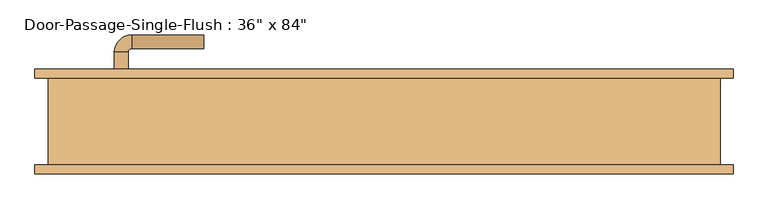
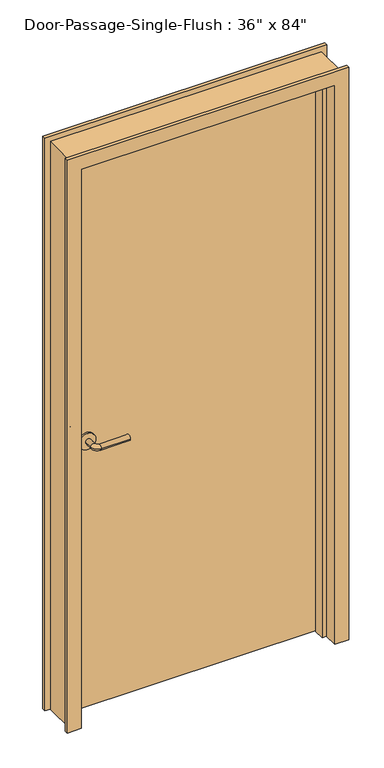
"""IFC4 building model written with IfcOpenShell, lengths in millimetres: door geometry."""

import ifcopenshell
import ifcopenshell.guid

model = None  # the IFC model being written
_history = None  # IfcOwnerHistory: only IFC2X3 demands one
_inside = {}  # id of a spatial element -> (the spatial element, [elements in it])
_under = {}  # id of a project, library or spatial element -> (it, [spatial elements below it])
_declared = {}  # id of a project -> (the project, [libraries it declares])
_typed = {}  # id of a type object -> (the type object, [elements of that type])
_made_of = {}  # id of a material, layer set ... -> (it, [elements and type objects made of it])


def new_model(schema):
    """Start an empty IFC model of exactly this schema.

    Asked for "IFC4X3", IfcOpenShell would pick the latest addendum, in which some entities
    have other attributes; the version numbers below select the first issue.
    IFC2X3 requires an IfcOwnerHistory on every rooted entity: one is made here for all.
    """
    global model, _history
    if schema == "IFC4X3":
        model = ifcopenshell.file(schema_version=(4, 3, 0, 0))
    else:
        model = ifcopenshell.file(schema=schema)
    _inside.clear()
    _under.clear()
    _declared.clear()
    _typed.clear()
    _made_of.clear()
    _history = None
    if model.schema == "IFC2X3":
        org = make("IfcOrganization", Name="unknown")
        user = make(
            "IfcPersonAndOrganization",
            ThePerson=make("IfcPerson", FamilyName="unknown"),
            TheOrganization=org,
        )
        app = make(
            "IfcApplication",
            ApplicationDeveloper=org,
            Version="unknown",
            ApplicationFullName="unknown",
            ApplicationIdentifier="unknown",
        )
        _history = make(
            "IfcOwnerHistory",
            OwningUser=user,
            OwningApplication=app,
            ChangeAction="ADDED",
            CreationDate=0,
        )
    return model


def make(cls, **values):
    """One entity of the class cls with the attributes given. An attribute that is None is left unset."""
    return model.create_entity(
        cls, **{name: value for name, value in values.items() if value is not None}
    )


def rooted(cls, **values):
    """An entity with a GlobalId (a new one), such as an element, a storey or a relation."""
    return make(cls, GlobalId=ifcopenshell.guid.new(), OwnerHistory=_history, **values)


def si_unit(unit_type, name, prefix=None):
    """IfcSIUnit, for example si_unit("LENGTHUNIT", "METRE", prefix="MILLI")."""
    return make("IfcSIUnit", UnitType=unit_type, Prefix=prefix, Name=name)


def assignment(units):
    """IfcUnitAssignment: the units of a project."""
    return None if units is None else make("IfcUnitAssignment", Units=units)


def point(xyz):
    """IfcCartesianPoint."""
    return None if xyz is None else make("IfcCartesianPoint", Coordinates=xyz)


def direction(xyz):
    """IfcDirection."""
    return None if xyz is None else make("IfcDirection", DirectionRatios=xyz)


def frame(location, z_axis=None, x_axis=None):
    """IfcAxis2Placement3D, a coordinate frame: its origin and axes. An axis left out is left unset."""
    return make(
        "IfcAxis2Placement3D",
        Location=point(location),
        Axis=direction(z_axis),
        RefDirection=direction(x_axis),
    )


def frame_2d(location, x_axis=None):
    """IfcAxis2Placement2D, a coordinate frame in the plane: its origin and x axis."""
    return make(
        "IfcAxis2Placement2D", Location=point(location), RefDirection=direction(x_axis)
    )


def origin():
    """The frame at (0, 0, 0) with its axes left unset."""
    return frame((0.0, 0.0, 0.0))


def origin_with_axes():
    """The frame at (0, 0, 0) with the z axis (0, 0, 1) and the x axis (1, 0, 0) written out."""
    return frame((0.0, 0.0, 0.0), z_axis=(0.0, 0.0, 1.0), x_axis=(1.0, 0.0, 0.0))


def place(relative_to, where):
    """IfcLocalPlacement: puts the frame where relative to a parent placement (None: the world)."""
    return make(
        "IfcLocalPlacement", PlacementRelTo=relative_to, RelativePlacement=where
    )


def context(
    kind, dimensions, precision=None, world=None, true_north=None, identifier=None
):
    """IfcGeometricRepresentationContext, for example the 3D "Model" context."""
    return make(
        "IfcGeometricRepresentationContext",
        ContextIdentifier=identifier,
        ContextType=kind,
        CoordinateSpaceDimension=dimensions,
        Precision=precision,
        WorldCoordinateSystem=world,
        TrueNorth=true_north,
    )


def project(units=None, contexts=None):
    """IfcProject with its units and contexts."""
    return rooted(
        "IfcProject",
        Name="project",
        RepresentationContexts=contexts,
        UnitsInContext=assignment(units),
    )


def spatial(cls, under=None, at=None, **own):
    """A site, building, storey or space (cls), placed at a placement, below another one or the project."""
    s = rooted(cls, ObjectPlacement=at, **own)
    if under is not None:
        _under.setdefault(under.id(), (under, []))[1].append(s)
    return s


def polyline(points):
    """IfcPolyline through the points."""
    return make("IfcPolyline", Points=[point(p) for p in points])


def circle_curve(where, radius):
    """IfcCircle in the frame where."""
    return make("IfcCircle", Position=where, Radius=radius)


def ellipse_curve(where, semi_axis1, semi_axis2):
    """IfcEllipse in the frame where."""
    return make(
        "IfcEllipse", Position=where, SemiAxis1=semi_axis1, SemiAxis2=semi_axis2
    )


def trimmed(basis, trim1, trim2, sense, master):
    """IfcTrimmedCurve: the piece of a basis curve between two trims."""
    return make(
        "IfcTrimmedCurve",
        BasisCurve=basis,
        Trim1=trim1,
        Trim2=trim2,
        SenseAgreement=sense,
        MasterRepresentation=master,
    )


def segment(curve, same_sense, transition):
    """IfcCompositeCurveSegment."""
    return make(
        "IfcCompositeCurveSegment",
        Transition=transition,
        SameSense=same_sense,
        ParentCurve=curve,
    )


def composite_curve(segments, self_intersect=None):
    """IfcCompositeCurve: segments joined end to end."""
    return make("IfcCompositeCurve", Segments=segments, SelfIntersect=self_intersect)


def outline(outer, holes=None, kind="AREA"):
    """IfcArbitraryClosedProfileDef: a profile drawn as a closed curve; with holes, ...WithVoids."""
    if holes is None:
        return make("IfcArbitraryClosedProfileDef", ProfileType=kind, OuterCurve=outer)
    return make(
        "IfcArbitraryProfileDefWithVoids",
        ProfileType=kind,
        OuterCurve=outer,
        InnerCurves=holes,
    )


def extrude(swept, where, along, depth):
    """IfcExtrudedAreaSolid: the profile swept, set in the frame where, extruded along a direction by depth."""
    return make(
        "IfcExtrudedAreaSolid",
        SweptArea=swept,
        Position=where,
        ExtrudedDirection=direction(along),
        Depth=depth,
    )


def faces_of(points, faces, orient=None, outer=None):
    """IfcFace entities. A face is a list of loops; a loop is a list of indices into points, from 0.

    orient and outer hold one flag for each loop. By default every Orientation is true, the
    first loop of a face is its IfcFaceOuterBound and the others are IfcFaceBound.
    """
    made = []
    for i, loops in enumerate(faces):
        bounds = []
        for j, loop in enumerate(loops):
            is_outer = j == 0 if outer is None else outer[i][j]
            bounds.append(
                make(
                    "IfcFaceOuterBound" if is_outer else "IfcFaceBound",
                    Bound=make("IfcPolyLoop", Polygon=[points[k] for k in loop]),
                    Orientation=True if orient is None else orient[i][j],
                )
            )
        made.append(make("IfcFace", Bounds=bounds))
    return made


def faceted_brep(points, faces, orient=None, outer=None, voids=None):
    """IfcFacetedBrep: a solid bounded by flat faces; with voids (closed shells), ...WithVoids."""
    shared = [point(p) for p in points]
    hull = make("IfcClosedShell", CfsFaces=faces_of(shared, faces, orient, outer))
    if voids is None:
        return make("IfcFacetedBrep", Outer=hull)
    return make(
        "IfcFacetedBrepWithVoids",
        Outer=hull,
        Voids=[
            make(cls, CfsFaces=faces_of(shared, fs, o, b)) for cls, fs, o, b in voids
        ],
    )


def shape(context_of_items, identifier, shape_type, items):
    """IfcShapeRepresentation: the items that make up one representation, for example the "Body"."""
    return make(
        "IfcShapeRepresentation",
        ContextOfItems=context_of_items,
        RepresentationIdentifier=identifier,
        RepresentationType=shape_type,
        Items=items,
    )


def source(mapping_origin, context_of_items, identifier, shape_type, items):
    """IfcRepresentationMap: a shape defined once, which mapped items show again and again."""
    return make(
        "IfcRepresentationMap",
        MappingOrigin=mapping_origin,
        MappedRepresentation=shape(context_of_items, identifier, shape_type, items),
    )


def transform(
    local_origin,
    x_axis=None,
    y_axis=None,
    z_axis=None,
    scale=None,
    scale2=None,
    scale3=None,
    uniform=True,
):
    """IfcCartesianTransformationOperator3D, or its non-uniform kind. x_axis, y_axis, z_axis: its Axis1, 2, 3."""
    if uniform:
        return make(
            "IfcCartesianTransformationOperator3D",
            Axis1=direction(x_axis),
            Axis2=direction(y_axis),
            LocalOrigin=point(local_origin),
            Scale=scale,
            Axis3=direction(z_axis),
        )
    return make(
        "IfcCartesianTransformationOperator3DnonUniform",
        Axis1=direction(x_axis),
        Axis2=direction(y_axis),
        LocalOrigin=point(local_origin),
        Scale=scale,
        Axis3=direction(z_axis),
        Scale2=scale2,
        Scale3=scale3,
    )


def mapped(mapping_source, mapping_target):
    """IfcMappedItem: shows the shape of a source again, moved by a transform."""
    return make(
        "IfcMappedItem", MappingSource=mapping_source, MappingTarget=mapping_target
    )


def made_of(thing, what):
    """Note that an element or type object is made of a material, layer set ...; save() writes the relation."""
    if what is not None:
        _made_of.setdefault(what.id(), (what, []))[1].append(thing)
    return thing


def element(
    cls,
    number,
    at=None,
    inside=None,
    cuts=None,
    type_object=None,
    material=None,
    context=None,
    identifier="Body",
    shape_type=None,
    held_by="IfcProductDefinitionShape",
    body=None,
    shapes=None,
    **own,
):
    """One element of the class cls, such as IfcWall. Its Tag is "e" and its number.

    at: its placement. inside: the storey or other place that contains it. cuts: it is an
    opening in that element (IfcRelVoidsElement). A single representation is given by context,
    identifier, shape_type and body (its items); several are given by shapes. held_by: the class
    of the entity that holds the representations. save() writes the other relations.
    """
    e = rooted(cls, Tag="e%d" % number, ObjectPlacement=at, **own)
    if body is not None:
        shapes = [shape(context, identifier, shape_type, body)]
    if shapes is not None:
        e.Representation = make(held_by, Representations=shapes)
    if inside is not None:
        _inside.setdefault(inside.id(), (inside, []))[1].append(e)
    if cuts is not None:
        rooted(
            "IfcRelVoidsElement", RelatingBuildingElement=cuts, RelatedOpeningElement=e
        )
    if type_object is not None:
        _typed.setdefault(type_object.id(), (type_object, []))[1].append(e)
    return made_of(e, material)


def aggregate(whole, parts):
    """IfcRelAggregates: a whole, such as a stair, and the parts it consists of."""
    return rooted("IfcRelAggregates", RelatingObject=whole, RelatedObjects=parts)


def save(model, path):
    """Write the relations noted so far, then the file.

    IfcRelAggregates (storeys below a building ...), IfcRelContainedInSpatialStructure (elements
    in a storey), IfcRelDefinesByType, IfcRelAssociatesMaterial and IfcRelDeclares: one each for
    every whole, place, type object, material and project.
    """
    for whole, parts in _under.values():
        aggregate(whole, parts)
    for where, things in _inside.values():
        rooted(
            "IfcRelContainedInSpatialStructure",
            RelatedElements=things,
            RelatingStructure=where,
        )
    for kind, things in _typed.values():
        rooted("IfcRelDefinesByType", RelatedObjects=things, RelatingType=kind)
    for what, things in _made_of.values():
        rooted("IfcRelAssociatesMaterial", RelatedObjects=things, RelatingMaterial=what)
    for by, libraries in _declared.values():
        rooted("IfcRelDeclares", RelatingContext=by, RelatedDefinitions=libraries)
    model.write(path)


def plane_surface(at):
    """IfcPlane: the flat surface through the origin of the frame at, square to its z axis."""
    return make("IfcPlane", Position=at)


def cylinder_surface(at, radius):
    """IfcCylindricalSurface: all points at the distance radius from the z axis of the frame at."""
    return make("IfcCylindricalSurface", Position=at, Radius=radius)


def revolved_surface(curve, axis_point, axis_direction):
    """IfcSurfaceOfRevolution: the curve turned about the line through axis_point along axis_direction."""
    return make(
        "IfcSurfaceOfRevolution",
        SweptCurve=make("IfcArbitraryOpenProfileDef", ProfileType="CURVE", Curve=curve),
        AxisPosition=make("IfcAxis1Placement", Location=point(axis_point), Axis=direction(axis_direction)),
    )


def advanced_brep(points, edges, surfaces, faces):
    """IfcAdvancedBrep: a solid bounded by faces that lie on surfaces and meet in shared edges.

    An edge is (start, end): straight between two places in points (the first is 0);
    or (start, end, curve); or (start, end, curve, False) where it runs against its curve.
    A face is (place in surfaces, loops), or (place, loops, False) where it looks against
    its surface's normal. A loop lists edges by number (the first is 1), with a minus sign
    where the edge is run from its end to its start. The first loop is the outer one.
    """
    corners = [point(p) for p in points]
    vertices = [make("IfcVertexPoint", VertexGeometry=c) for c in corners]
    made = []
    for start, end, *more in edges:
        made.append(
            make(
                "IfcEdgeCurve",
                EdgeStart=vertices[start],
                EdgeEnd=vertices[end],
                EdgeGeometry=more[0] if more else make("IfcPolyline", Points=[corners[start], corners[end]]),
                SameSense=more[1] if len(more) > 1 else True,
            )
        )
    hull = []
    for where, loops, *sense in faces:
        bounds = []
        for j, loop in enumerate(loops):
            ring = [make("IfcOrientedEdge", EdgeElement=made[abs(k) - 1], Orientation=k > 0) for k in loop]
            bounds.append(
                make(
                    "IfcFaceOuterBound" if j == 0 else "IfcFaceBound",
                    Bound=make("IfcEdgeLoop", EdgeList=ring),
                    Orientation=True,
                )
            )
        hull.append(make("IfcAdvancedFace", Bounds=bounds, FaceSurface=surfaces[where], SameSense=sense[0] if sense else True))
    return make("IfcAdvancedBrep", Outer=make("IfcClosedShell", CfsFaces=hull))


def door_12b10c6a(model_context):
    return source(origin(), model_context, "Body", "SolidModel", [
        advanced_brep(
        [(-392.190625, 17.4, 1016.0), (-372.190625, 17.4, 1016.0), (-372.190625, -12.6, 1016.0), (-392.190625, -12.6, 1016.0), (-367.190625, -17.6, 1016.0), (-367.190625, -37.6, 1016.0), (-262.190625, -37.6, 1016.0), (-262.190625, -17.6, 1016.0)],
        [
            (0, 1, circle_curve(frame((-382.190625, 17.4, 1016.0), z_axis=(0.0, 1.0, 0.0), x_axis=(1.0, 0.0, 0.0)), 10.0)),
            (1, 0, circle_curve(frame((-382.190625, 17.4, 1016.0), z_axis=(0.0, 1.0, 0.0), x_axis=(1.0, 0.0, 0.0)), 10.0)),
            (1, 2),
            (2, 3, circle_curve(frame((-382.190625, -12.6, 1016.0), z_axis=(0.0, 1.0, 0.0), x_axis=(1.0, 0.0, 0.0)), 10.0)),
            (3, 0),
            (3, 2, circle_curve(frame((-382.190625, -12.6, 1016.0), z_axis=(0.0, 1.0, 0.0), x_axis=(1.0, 0.0, 0.0)), 10.0)),
            (4, 5, circle_curve(frame((-367.190625, -27.6, 1016.0), z_axis=(-1.0, 0.0, 0.0), x_axis=(0.0, 1.0, 0.0)), 10.0)),
            (5, 3, circle_curve(frame((-367.190625, -12.6, 1016.0), z_axis=(0.0, 0.0, -1.0), x_axis=(-1.0, 0.0, 0.0)), 25.0)),
            (2, 4, circle_curve(frame((-367.190625, -12.6, 1016.0), z_axis=(0.0, 0.0, 1.0), x_axis=(-1.0, 0.0, 0.0)), 5.0)),
            (5, 4, circle_curve(frame((-367.190625, -27.6, 1016.0), z_axis=(-1.0, 0.0, 0.0), x_axis=(0.0, 1.0, 0.0)), 10.0)),
            (6, 7, circle_curve(frame((-262.190625, -27.6, 1016.0), z_axis=(1.0, 0.0, 0.0), x_axis=(0.0, 1.0, 0.0)), 10.0)),
            (7, 6, circle_curve(frame((-262.190625, -27.6, 1016.0), z_axis=(1.0, 0.0, 0.0), x_axis=(0.0, 1.0, 0.0)), 10.0)),
            (4, 7),
            (6, 5),
        ],
        [
            plane_surface(frame((-382.190625, 17.4, 1016.0), z_axis=(0.0, 1.0, 0.0), x_axis=(0.0, 0.0, 1.0))),
            cylinder_surface(frame((-382.190625, 17.4, 1016.0), z_axis=(0.0, 1.0, 0.0), x_axis=(1.0, 0.0, 0.0)), 10.0),
            revolved_surface(trimmed(ellipse_curve(frame((-382.190625, -12.6, 1016.0), z_axis=(0.0, -1.0, 0.0), x_axis=(1.0, 0.0, 0.0)), 10.0, 10.0), [point((-392.190625, -12.6, 1016.0))], [point((-372.190625, -12.6, 1016.0))], True, "CARTESIAN"), (-367.190625, -12.6, 1016.0), (0.0, 0.0, -1.0)),
            revolved_surface(trimmed(ellipse_curve(frame((-382.190625, -12.6, 1016.0), z_axis=(0.0, -1.0, 0.0), x_axis=(1.0, 0.0, 0.0)), 10.0, 10.0), [point((-372.190625, -12.6, 1016.0))], [point((-392.190625, -12.6, 1016.0))], True, "CARTESIAN"), (-367.190625, -12.6, 1016.0), (0.0, 0.0, -1.0)),
            plane_surface(frame((-262.190625, -27.6, 1016.0), z_axis=(1.0, 0.0, 0.0), x_axis=(0.0, 0.0, 1.0))),
            cylinder_surface(frame((-367.190625, -27.6, 1016.0), z_axis=(-1.0, 0.0, 0.0), x_axis=(0.0, 1.0, 0.0)), 10.0),
        ],
        [
            (0, [[1, 2]]),
            (1, [[3, 4, 5, -2]]),
            (1, [[-5, 6, -3, -1]]),
            (2, [[7, 8, -4, 9]]),
            (3, [[10, -9, -6, -8]]),
            (4, [[11, 12]]),
            (5, [[13, -11, 14, -7]]),
            (5, [[-14, -12, -13, -10]]),
        ],
    ),
        extrude(outline(composite_curve([segment(trimmed(circle_curve(frame_2d((1016.0, -384.690625)), 30.0), [point((1016.0, -414.690625))], [point((1016.0, -354.690625))], False, "CARTESIAN"), True, "CONTINUOUS"), segment(trimmed(circle_curve(frame_2d((1016.0, -384.690625)), 30.0), [point((1016.0, -354.690625))], [point((1016.0, -414.690625))], False, "CARTESIAN"), True, "CONTINUOUS")], self_intersect=False)), frame((0.0, 17.4, 0.0), z_axis=(0.0, 1.0, 0.0), x_axis=(0.0, 0.0, 1.0)), (0.0, 0.0, 1.0), 8.0),
        advanced_brep(
        [(-392.190625, 77.85, 1016.0), (-372.190625, 77.85, 1016.0), (-392.190625, 107.85, 1016.0), (-372.190625, 107.85, 1016.0), (-367.190625, 112.85, 1016.0), (-367.190625, 132.85, 1016.0), (-262.190625, 132.85, 1016.0), (-262.190625, 112.85, 1016.0)],
        [
            (0, 1, circle_curve(frame((-382.190625, 77.85, 1016.0), z_axis=(0.0, -1.0, 0.0), x_axis=(1.0, 0.0, 0.0)), 10.0)),
            (1, 0, circle_curve(frame((-382.190625, 77.85, 1016.0), z_axis=(0.0, -1.0, 0.0), x_axis=(1.0, 0.0, 0.0)), 10.0)),
            (0, 2),
            (2, 3, circle_curve(frame((-382.190625, 107.85, 1016.0), z_axis=(0.0, -1.0, 0.0), x_axis=(1.0, 0.0, 0.0)), 10.0)),
            (3, 1),
            (3, 2, circle_curve(frame((-382.190625, 107.85, 1016.0), z_axis=(0.0, -1.0, 0.0), x_axis=(1.0, 0.0, 0.0)), 10.0)),
            (4, 3, circle_curve(frame((-367.190625, 107.85, 1016.0), z_axis=(0.0, 0.0, 1.0), x_axis=(-1.0, 0.0, 0.0)), 5.0)),
            (2, 5, circle_curve(frame((-367.190625, 107.85, 1016.0), z_axis=(0.0, 0.0, -1.0), x_axis=(-1.0, 0.0, 0.0)), 25.0)),
            (5, 4, circle_curve(frame((-367.190625, 122.85, 1016.0), z_axis=(-1.0, 0.0, 0.0), x_axis=(0.0, -1.0, 0.0)), 10.0)),
            (4, 5, circle_curve(frame((-367.190625, 122.85, 1016.0), z_axis=(-1.0, 0.0, 0.0), x_axis=(0.0, -1.0, 0.0)), 10.0)),
            (6, 7, circle_curve(frame((-262.190625, 122.85, 1016.0), z_axis=(1.0, 0.0, 0.0), x_axis=(0.0, -1.0, 0.0)), 10.0)),
            (7, 6, circle_curve(frame((-262.190625, 122.85, 1016.0), z_axis=(1.0, 0.0, 0.0), x_axis=(0.0, -1.0, 0.0)), 10.0)),
            (5, 6),
            (7, 4),
        ],
        [
            plane_surface(frame((-382.190625, 77.85, 1016.0), z_axis=(0.0, -1.0, 0.0), x_axis=(0.0, 0.0, 1.0))),
            cylinder_surface(frame((-382.190625, 77.85, 1016.0), z_axis=(0.0, -1.0, 0.0), x_axis=(1.0, 0.0, 0.0)), 10.0),
            revolved_surface(trimmed(ellipse_curve(frame((-382.190625, 107.85, 1016.0), z_axis=(0.0, -1.0, 0.0), x_axis=(1.0, 0.0, 0.0)), 10.0, 10.0), [point((-392.190625, 107.85, 1016.0))], [point((-372.190625, 107.85, 1016.0))], True, "CARTESIAN"), (-367.190625, 107.85, 1016.0), (0.0, 0.0, -1.0)),
            revolved_surface(trimmed(ellipse_curve(frame((-382.190625, 107.85, 1016.0), z_axis=(0.0, -1.0, 0.0), x_axis=(1.0, 0.0, 0.0)), 10.0, 10.0), [point((-372.190625, 107.85, 1016.0))], [point((-392.190625, 107.85, 1016.0))], True, "CARTESIAN"), (-367.190625, 107.85, 1016.0), (0.0, 0.0, -1.0)),
            plane_surface(frame((-262.190625, 122.85, 1016.0), z_axis=(1.0, 0.0, 0.0), x_axis=(0.0, 0.0, 1.0))),
            cylinder_surface(frame((-367.190625, 122.85, 1016.0), z_axis=(-1.0, 0.0, 0.0), x_axis=(0.0, -1.0, 0.0)), 10.0),
        ],
        [
            (0, [[1, 2]]),
            (1, [[-1, 3, 4, 5]]),
            (1, [[-2, -5, 6, -3]]),
            (2, [[7, -4, 8, 9]]),
            (3, [[-8, -6, -7, 10]]),
            (4, [[11, 12]]),
            (5, [[-9, 13, -12, 14]]),
            (5, [[-10, -14, -11, -13]]),
        ],
    ),
        extrude(outline(composite_curve([segment(trimmed(circle_curve(frame_2d((1016.0, -384.690625)), 30.0), [point((1016.0, -414.690625))], [point((1016.0, -354.690625))], False, "CARTESIAN"), True, "CONTINUOUS"), segment(trimmed(circle_curve(frame_2d((1016.0, -384.690625)), 30.0), [point((1016.0, -354.690625))], [point((1016.0, -414.690625))], False, "CARTESIAN"), True, "CONTINUOUS")], self_intersect=False)), frame((0.0, 69.85, 0.0), z_axis=(0.0, 1.0, 0.0), x_axis=(0.0, 0.0, 1.0)), (0.0, 0.0, 1.0), 8.0),
        faceted_brep([(457.2, 82.55, 0.0), (508.0, 82.55, 0.0), (508.0, 69.85, 0.0), (488.95, 69.85, 0.0), (488.95, -57.15, 0.0), (508.0, -57.15, 0.0), (508.0, -69.85, 0.0), (457.2, -69.85, 0.0), (457.2, -17.4625, 0.0), (441.325, -17.4625, 0.0), (441.325, 20.6375, 0.0), (457.2, 20.6375, 0.0), (457.2, 82.55, 2133.6), (-457.2, 82.55, 2133.6), (-457.2, 82.55, 0.0), (-508.0, 82.55, 0.0), (-508.0, 82.55, 2184.4), (508.0, 82.55, 2184.4), (508.0, 69.85, 2184.4), (-508.0, 69.85, 2184.4), (-508.0, 69.85, 0.0), (-488.95, 69.85, 0.0), (-488.95, 69.85, 2165.35), (488.95, 69.85, 2165.35), (488.95, -57.15, 2165.35), (-488.95, -57.15, 2165.35), (-488.95, -57.15, 0.0), (-508.0, -57.15, 0.0), (-508.0, -57.15, 2184.4), (508.0, -57.15, 2184.4), (508.0, -69.85, 2184.4), (-508.0, -69.85, 2184.4), (-508.0, -69.85, 0.0), (-457.2, -69.85, 0.0), (-457.2, -69.85, 2133.6), (457.2, -69.85, 2133.6), (457.2, -17.4625, 2133.6), (-457.2, -17.4625, 2133.6), (-457.2, -17.4625, 0.0), (-441.325, -17.4625, 0.0), (-441.325, -17.4625, 2117.725), (441.325, -17.4625, 2117.725), (441.325, 20.6375, 2117.725), (-441.325, 20.6375, 2117.725), (-441.325, 20.6375, 0.0), (-457.2, 20.6375, 0.0), (-457.2, 20.6375, 2133.6), (457.2, 20.6375, 2133.6)], [[[0, 1, 2, 3, 4, 5, 6, 7, 8, 9, 10, 11]], [[1, 0, 12, 13, 14, 15, 16, 17]], [[2, 1, 17, 18]], [[3, 2, 18, 19, 20, 21, 22, 23]], [[4, 3, 23, 24]], [[5, 4, 24, 25, 26, 27, 28, 29]], [[6, 5, 29, 30]], [[7, 6, 30, 31, 32, 33, 34, 35]], [[8, 7, 35, 36]], [[9, 8, 36, 37, 38, 39, 40, 41]], [[10, 9, 41, 42]], [[11, 10, 42, 43, 44, 45, 46, 47]], [[0, 11, 47, 12]], [[18, 17, 16, 19]], [[24, 23, 22, 25]], [[30, 29, 28, 31]], [[36, 35, 34, 37]], [[42, 41, 40, 43]], [[12, 47, 46, 13]], [[14, 45, 44, 39, 38, 33, 32, 27, 26, 21, 20, 15]], [[19, 16, 15, 20]], [[25, 22, 21, 26]], [[31, 28, 27, 32]], [[37, 34, 33, 38]], [[43, 40, 39, 44]], [[13, 46, 45, 14]]]),
        extrude(outline(polyline([(457.2, 25.4), (-457.2, 25.4), (-457.2, 69.85), (457.2, 69.85), (457.2, 25.4)])), origin_with_axes(), (0.0, 0.0, 1.0), 2133.6),
    ])


if __name__ == "__main__":
    model = new_model("IFC4")
    model_context = context("Model", 3, world=origin())
    ifc_project = project(units=[si_unit("LENGTHUNIT", "METRE", prefix="MILLI")], contexts=[model_context])
    site = spatial("IfcSite", under=ifc_project)
    building = spatial("IfcBuilding", under=site)
    placement = place(None, origin())
    door_shape = door_12b10c6a(model_context)
    element("IfcDoor", 1, ObjectType="Door-Passage-Single-Flush : 36\" x 84\"", at=placement, inside=building, context=model_context, shape_type="MappedRepresentation", body=[
        mapped(door_shape, transform((0.0, 0.0, 0.0), x_axis=(1.0, 0.0, 0.0), y_axis=(0.0, 1.0, 0.0), z_axis=(0.0, 0.0, 1.0))),
    ])
    save(model, "model.ifc")

# Revit data of these elements
# Type "Door-Passage-Single-Flush : 36\" x 84\""
#   Type Mark = "19"
#   Fire Rating = "--"
#   Assembly Code = "B2030200"
#   Analytic Construction = "Wooden"
#   Thickness = 0' - 1 3/4"
#   Thermal Resistance (R) = 2.5876 (h·ft²·°F)/BTU
#   Swing Angle [instance default] = 90.00°
#   Strike Height = 3' - 4"
#   Rough Width [instance default] = 3' - 4"
#   Rough Height [instance default] = 7' - 4"
#   MF Opening Height [instance default] = 0' - 4"
#   MF Opening Width [instance default] = 0' - 4"
#   Inset Calculate [instance default] = 0' - 4"
#   Masonry Inset [instance default] = 0' - 1"
#   Height = 7' - 0"
#   Width = 3' - 0"
#   Heat Transfer Coefficient (U) = 0.3865 BTU/(h·ft²·°F)
#   Masonry Frame Depth = 0' - 5 3/4"
#   Masonry Frame [instance default] = yes
#   Function = 1
#   Dry Wall Frame [instance default] = no
#   Panel Material = Wood - Birch
#   Frame Material = Metal - Paint Finish - Grey
#   Door Handle Material = Aluminum
#   Visual Light Transmittance = 0
#   Solar Heat Gain Coefficient = 0
#   Wall Closure = (empty or 0)
# Element 1 (IfcDoor, "Door-Passage-Single-Flush : 36\" x 84\"")
#   Rough Width = 3' - 2 1/2"
#   Rough Height = 7' - 1 1/4"
#   MF Opening Height = 0' - 1 1/4"
#   MF Opening Width = 0' - 2 1/2"
#   Inset Calculate = 0' - 3"
#   Masonry Frame = no
#   Dry Wall Frame = yes
#   Materials on its faces: "Metal - Paint Finish - Grey", "Aluminum", "Wood - Birch"
# Materials
#   "Wood - Birch": class "Wood", colour RGB 166 116 52, transparency 0, Cost = 0
#   "Metal - Paint Finish - Grey": class "Paint", colour RGB 104 104 104, transparency 0, Cost = 0
#   "Aluminum": class "Metal", colour RGB 247 247 247, transparency 0, Description = "Aluminum 6061", Cost = 0
